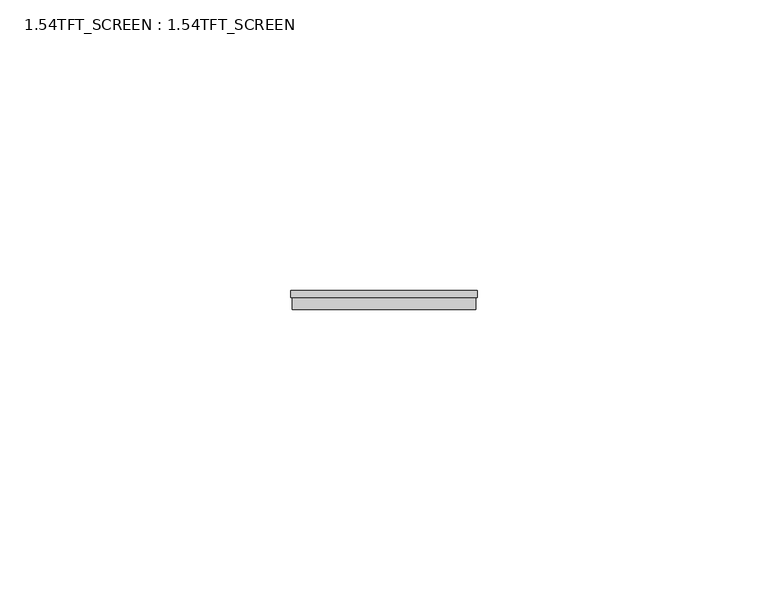
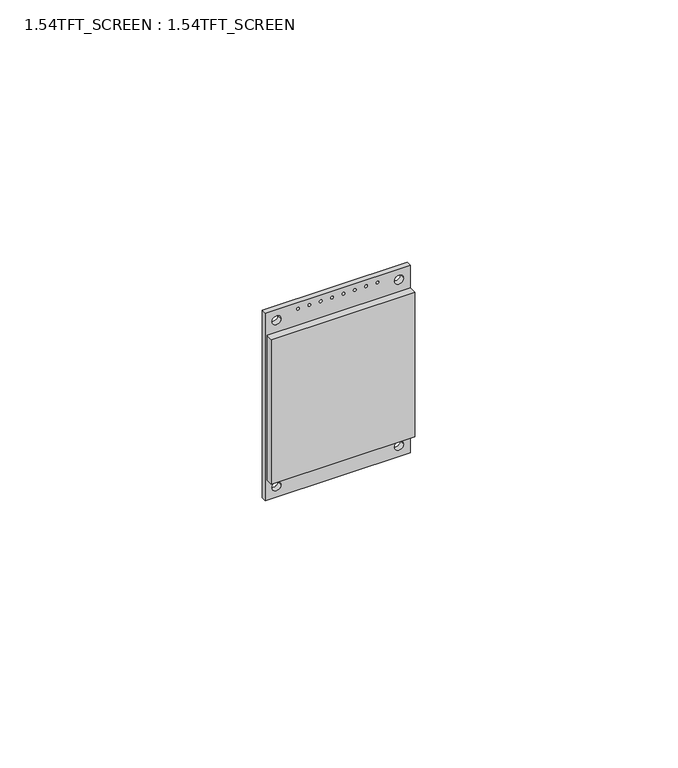
"""IFC4 building model written with IfcOpenShell, lengths in millimetres: furniture geometry, 1.54TFT_SCREEN : 1.54TFT_SCREEN."""

import ifcopenshell
import ifcopenshell.guid

model = None  # the IFC model being written
_history = None  # IfcOwnerHistory: only IFC2X3 demands one
_inside = {}  # id of a spatial element -> (the spatial element, [elements in it])
_under = {}  # id of a project, library or spatial element -> (it, [spatial elements below it])
_declared = {}  # id of a project -> (the project, [libraries it declares])
_typed = {}  # id of a type object -> (the type object, [elements of that type])
_made_of = {}  # id of a material, layer set ... -> (it, [elements and type objects made of it])


def new_model(schema):
    """Start an empty IFC model of exactly this schema.

    Asked for "IFC4X3", IfcOpenShell would pick the latest addendum, in which some entities
    have other attributes; the version numbers below select the first issue.
    IFC2X3 requires an IfcOwnerHistory on every rooted entity: one is made here for all.
    """
    global model, _history
    if schema == "IFC4X3":
        model = ifcopenshell.file(schema_version=(4, 3, 0, 0))
    else:
        model = ifcopenshell.file(schema=schema)
    _inside.clear()
    _under.clear()
    _declared.clear()
    _typed.clear()
    _made_of.clear()
    _history = None
    if model.schema == "IFC2X3":
        org = make("IfcOrganization", Name="unknown")
        user = make(
            "IfcPersonAndOrganization",
            ThePerson=make("IfcPerson", FamilyName="unknown"),
            TheOrganization=org,
        )
        app = make(
            "IfcApplication",
            ApplicationDeveloper=org,
            Version="unknown",
            ApplicationFullName="unknown",
            ApplicationIdentifier="unknown",
        )
        _history = make(
            "IfcOwnerHistory",
            OwningUser=user,
            OwningApplication=app,
            ChangeAction="ADDED",
            CreationDate=0,
        )
    return model


def make(cls, **values):
    """One entity of the class cls with the attributes given. An attribute that is None is left unset."""
    return model.create_entity(
        cls, **{name: value for name, value in values.items() if value is not None}
    )


def rooted(cls, **values):
    """An entity with a GlobalId (a new one), such as an element, a storey or a relation."""
    return make(cls, GlobalId=ifcopenshell.guid.new(), OwnerHistory=_history, **values)


def si_unit(unit_type, name, prefix=None):
    """IfcSIUnit, for example si_unit("LENGTHUNIT", "METRE", prefix="MILLI")."""
    return make("IfcSIUnit", UnitType=unit_type, Prefix=prefix, Name=name)


def assignment(units):
    """IfcUnitAssignment: the units of a project."""
    return None if units is None else make("IfcUnitAssignment", Units=units)


def point(xyz):
    """IfcCartesianPoint."""
    return None if xyz is None else make("IfcCartesianPoint", Coordinates=xyz)


def direction(xyz):
    """IfcDirection."""
    return None if xyz is None else make("IfcDirection", DirectionRatios=xyz)


def frame(location, z_axis=None, x_axis=None):
    """IfcAxis2Placement3D, a coordinate frame: its origin and axes. An axis left out is left unset."""
    return make(
        "IfcAxis2Placement3D",
        Location=point(location),
        Axis=direction(z_axis),
        RefDirection=direction(x_axis),
    )


def frame_2d(location, x_axis=None):
    """IfcAxis2Placement2D, a coordinate frame in the plane: its origin and x axis."""
    return make(
        "IfcAxis2Placement2D", Location=point(location), RefDirection=direction(x_axis)
    )


def origin():
    """The frame at (0, 0, 0) with its axes left unset."""
    return frame((0.0, 0.0, 0.0))


def place(relative_to, where):
    """IfcLocalPlacement: puts the frame where relative to a parent placement (None: the world)."""
    return make(
        "IfcLocalPlacement", PlacementRelTo=relative_to, RelativePlacement=where
    )


def context(
    kind, dimensions, precision=None, world=None, true_north=None, identifier=None
):
    """IfcGeometricRepresentationContext, for example the 3D "Model" context."""
    return make(
        "IfcGeometricRepresentationContext",
        ContextIdentifier=identifier,
        ContextType=kind,
        CoordinateSpaceDimension=dimensions,
        Precision=precision,
        WorldCoordinateSystem=world,
        TrueNorth=true_north,
    )


def project(units=None, contexts=None):
    """IfcProject with its units and contexts."""
    return rooted(
        "IfcProject",
        Name="project",
        RepresentationContexts=contexts,
        UnitsInContext=assignment(units),
    )


def spatial(cls, under=None, at=None, **own):
    """A site, building, storey or space (cls), placed at a placement, below another one or the project."""
    s = rooted(cls, ObjectPlacement=at, **own)
    if under is not None:
        _under.setdefault(under.id(), (under, []))[1].append(s)
    return s


def polyline(points):
    """IfcPolyline through the points."""
    return make("IfcPolyline", Points=[point(p) for p in points])


def circle_curve(where, radius):
    """IfcCircle in the frame where."""
    return make("IfcCircle", Position=where, Radius=radius)


def trimmed(basis, trim1, trim2, sense, master):
    """IfcTrimmedCurve: the piece of a basis curve between two trims."""
    return make(
        "IfcTrimmedCurve",
        BasisCurve=basis,
        Trim1=trim1,
        Trim2=trim2,
        SenseAgreement=sense,
        MasterRepresentation=master,
    )


def segment(curve, same_sense, transition):
    """IfcCompositeCurveSegment."""
    return make(
        "IfcCompositeCurveSegment",
        Transition=transition,
        SameSense=same_sense,
        ParentCurve=curve,
    )


def composite_curve(segments, self_intersect=None):
    """IfcCompositeCurve: segments joined end to end."""
    return make("IfcCompositeCurve", Segments=segments, SelfIntersect=self_intersect)


def outline(outer, holes=None, kind="AREA"):
    """IfcArbitraryClosedProfileDef: a profile drawn as a closed curve; with holes, ...WithVoids."""
    if holes is None:
        return make("IfcArbitraryClosedProfileDef", ProfileType=kind, OuterCurve=outer)
    return make(
        "IfcArbitraryProfileDefWithVoids",
        ProfileType=kind,
        OuterCurve=outer,
        InnerCurves=holes,
    )


def extrude(swept, where, along, depth):
    """IfcExtrudedAreaSolid: the profile swept, set in the frame where, extruded along a direction by depth."""
    return make(
        "IfcExtrudedAreaSolid",
        SweptArea=swept,
        Position=where,
        ExtrudedDirection=direction(along),
        Depth=depth,
    )


def shape(context_of_items, identifier, shape_type, items):
    """IfcShapeRepresentation: the items that make up one representation, for example the "Body"."""
    return make(
        "IfcShapeRepresentation",
        ContextOfItems=context_of_items,
        RepresentationIdentifier=identifier,
        RepresentationType=shape_type,
        Items=items,
    )


def source(mapping_origin, context_of_items, identifier, shape_type, items):
    """IfcRepresentationMap: a shape defined once, which mapped items show again and again."""
    return make(
        "IfcRepresentationMap",
        MappingOrigin=mapping_origin,
        MappedRepresentation=shape(context_of_items, identifier, shape_type, items),
    )


def transform(
    local_origin,
    x_axis=None,
    y_axis=None,
    z_axis=None,
    scale=None,
    scale2=None,
    scale3=None,
    uniform=True,
):
    """IfcCartesianTransformationOperator3D, or its non-uniform kind. x_axis, y_axis, z_axis: its Axis1, 2, 3."""
    if uniform:
        return make(
            "IfcCartesianTransformationOperator3D",
            Axis1=direction(x_axis),
            Axis2=direction(y_axis),
            LocalOrigin=point(local_origin),
            Scale=scale,
            Axis3=direction(z_axis),
        )
    return make(
        "IfcCartesianTransformationOperator3DnonUniform",
        Axis1=direction(x_axis),
        Axis2=direction(y_axis),
        LocalOrigin=point(local_origin),
        Scale=scale,
        Axis3=direction(z_axis),
        Scale2=scale2,
        Scale3=scale3,
    )


def mapped(mapping_source, mapping_target):
    """IfcMappedItem: shows the shape of a source again, moved by a transform."""
    return make(
        "IfcMappedItem", MappingSource=mapping_source, MappingTarget=mapping_target
    )


def made_of(thing, what):
    """Note that an element or type object is made of a material, layer set ...; save() writes the relation."""
    if what is not None:
        _made_of.setdefault(what.id(), (what, []))[1].append(thing)
    return thing


def element(
    cls,
    number,
    at=None,
    inside=None,
    cuts=None,
    type_object=None,
    material=None,
    context=None,
    identifier="Body",
    shape_type=None,
    held_by="IfcProductDefinitionShape",
    body=None,
    shapes=None,
    **own,
):
    """One element of the class cls, such as IfcWall. Its Tag is "e" and its number.

    at: its placement. inside: the storey or other place that contains it. cuts: it is an
    opening in that element (IfcRelVoidsElement). A single representation is given by context,
    identifier, shape_type and body (its items); several are given by shapes. held_by: the class
    of the entity that holds the representations. save() writes the other relations.
    """
    e = rooted(cls, Tag="e%d" % number, ObjectPlacement=at, **own)
    if body is not None:
        shapes = [shape(context, identifier, shape_type, body)]
    if shapes is not None:
        e.Representation = make(held_by, Representations=shapes)
    if inside is not None:
        _inside.setdefault(inside.id(), (inside, []))[1].append(e)
    if cuts is not None:
        rooted(
            "IfcRelVoidsElement", RelatingBuildingElement=cuts, RelatedOpeningElement=e
        )
    if type_object is not None:
        _typed.setdefault(type_object.id(), (type_object, []))[1].append(e)
    return made_of(e, material)


def aggregate(whole, parts):
    """IfcRelAggregates: a whole, such as a stair, and the parts it consists of."""
    return rooted("IfcRelAggregates", RelatingObject=whole, RelatedObjects=parts)


def save(model, path):
    """Write the relations noted so far, then the file.

    IfcRelAggregates (storeys below a building ...), IfcRelContainedInSpatialStructure (elements
    in a storey), IfcRelDefinesByType, IfcRelAssociatesMaterial and IfcRelDeclares: one each for
    every whole, place, type object, material and project.
    """
    for whole, parts in _under.values():
        aggregate(whole, parts)
    for where, things in _inside.values():
        rooted(
            "IfcRelContainedInSpatialStructure",
            RelatedElements=things,
            RelatingStructure=where,
        )
    for kind, things in _typed.values():
        rooted("IfcRelDefinesByType", RelatedObjects=things, RelatingType=kind)
    for what, things in _made_of.values():
        rooted("IfcRelAssociatesMaterial", RelatedObjects=things, RelatingMaterial=what)
    for by, libraries in _declared.values():
        rooted("IfcRelDeclares", RelatingContext=by, RelatedDefinitions=libraries)
    model.write(path)


def furniture_1_54tft_screen_1_54tft_screen_d9e98271(model_context):
    return source(origin(), model_context, "Body", "SweptSolid", [
        extrude(outline(polyline([(43.7, 16.0), (43.7, -16.0), (0.0, -16.0), (0.0, 16.0), (43.7, 16.0)]), holes=[composite_curve([segment(trimmed(circle_curve(frame_2d((2.5, 13.5)), 1.0), [point((2.5, 14.5))], [point((2.5, 12.5))], True, "CARTESIAN"), True, "CONTINUOUS"), segment(trimmed(circle_curve(frame_2d((2.5, 13.5)), 1.0), [point((2.5, 12.5))], [point((2.5, 14.5))], True, "CARTESIAN"), True, "CONTINUOUS")], self_intersect=False), composite_curve([segment(trimmed(circle_curve(frame_2d((41.2, 13.5)), 1.0), [point((41.2, 14.5))], [point((41.2, 12.5))], True, "CARTESIAN"), True, "CONTINUOUS"), segment(trimmed(circle_curve(frame_2d((41.2, 13.5)), 1.0), [point((41.2, 12.5))], [point((41.2, 14.5))], True, "CARTESIAN"), True, "CONTINUOUS")], self_intersect=False), composite_curve([segment(trimmed(circle_curve(frame_2d((42.2, -1.25)), 0.3), [point((42.2, -0.95))], [point((42.2, -1.55))], True, "CARTESIAN"), True, "CONTINUOUS"), segment(trimmed(circle_curve(frame_2d((42.2, -1.25)), 0.3), [point((42.2, -1.55))], [point((42.2, -0.95))], True, "CARTESIAN"), True, "CONTINUOUS")], self_intersect=False), composite_curve([segment(trimmed(circle_curve(frame_2d((42.2, 1.25)), 0.3), [point((42.2, 1.55))], [point((42.2, 0.95))], True, "CARTESIAN"), True, "CONTINUOUS"), segment(trimmed(circle_curve(frame_2d((42.2, 1.25)), 0.3), [point((42.2, 0.95))], [point((42.2, 1.55))], True, "CARTESIAN"), True, "CONTINUOUS")], self_intersect=False), composite_curve([segment(trimmed(circle_curve(frame_2d((42.2, 3.75)), 0.3), [point((42.2, 4.05))], [point((42.2, 3.45))], True, "CARTESIAN"), True, "CONTINUOUS"), segment(trimmed(circle_curve(frame_2d((42.2, 3.75)), 0.3), [point((42.2, 3.45))], [point((42.2, 4.05))], True, "CARTESIAN"), True, "CONTINUOUS")], self_intersect=False), composite_curve([segment(trimmed(circle_curve(frame_2d((42.2, 6.25)), 0.3), [point((42.2, 6.55))], [point((42.2, 5.95))], True, "CARTESIAN"), True, "CONTINUOUS"), segment(trimmed(circle_curve(frame_2d((42.2, 6.25)), 0.3), [point((42.2, 5.95))], [point((42.2, 6.55))], True, "CARTESIAN"), True, "CONTINUOUS")], self_intersect=False), composite_curve([segment(trimmed(circle_curve(frame_2d((42.2, 8.75)), 0.3), [point((42.2, 9.05))], [point((42.2, 8.45))], True, "CARTESIAN"), True, "CONTINUOUS"), segment(trimmed(circle_curve(frame_2d((42.2, 8.75)), 0.3), [point((42.2, 8.45))], [point((42.2, 9.05))], True, "CARTESIAN"), True, "CONTINUOUS")], self_intersect=False), composite_curve([segment(trimmed(circle_curve(frame_2d((42.2, -3.75)), 0.3), [point((42.2, -3.45))], [point((42.2, -4.05))], True, "CARTESIAN"), True, "CONTINUOUS"), segment(trimmed(circle_curve(frame_2d((42.2, -3.75)), 0.3), [point((42.2, -4.05))], [point((42.2, -3.45))], True, "CARTESIAN"), True, "CONTINUOUS")], self_intersect=False), composite_curve([segment(trimmed(circle_curve(frame_2d((42.2, -6.25)), 0.3), [point((42.2, -5.95))], [point((42.2, -6.55))], True, "CARTESIAN"), True, "CONTINUOUS"), segment(trimmed(circle_curve(frame_2d((42.2, -6.25)), 0.3), [point((42.2, -6.55))], [point((42.2, -5.95))], True, "CARTESIAN"), True, "CONTINUOUS")], self_intersect=False), composite_curve([segment(trimmed(circle_curve(frame_2d((42.2, -8.75)), 0.3), [point((42.2, -8.45))], [point((42.2, -9.05))], True, "CARTESIAN"), True, "CONTINUOUS"), segment(trimmed(circle_curve(frame_2d((42.2, -8.75)), 0.3), [point((42.2, -9.05))], [point((42.2, -8.45))], True, "CARTESIAN"), True, "CONTINUOUS")], self_intersect=False), composite_curve([segment(trimmed(circle_curve(frame_2d((41.2, -13.5)), 1.0), [point((41.2, -14.5))], [point((41.2, -12.5))], True, "CARTESIAN"), True, "CONTINUOUS"), segment(trimmed(circle_curve(frame_2d((41.2, -13.5)), 1.0), [point((41.2, -12.5))], [point((41.2, -14.5))], True, "CARTESIAN"), True, "CONTINUOUS")], self_intersect=False), composite_curve([segment(trimmed(circle_curve(frame_2d((2.5, -13.5)), 1.0), [point((2.5, -14.5))], [point((2.5, -12.5))], True, "CARTESIAN"), True, "CONTINUOUS"), segment(trimmed(circle_curve(frame_2d((2.5, -13.5)), 1.0), [point((2.5, -12.5))], [point((2.5, -14.5))], True, "CARTESIAN"), True, "CONTINUOUS")], self_intersect=False)]), frame((0.0, -1.2, 0.0), z_axis=(0.0, 1.0, 0.0), x_axis=(0.0, 0.0, 1.0)), (0.0, 0.0, 1.0), 1.2),
        extrude(outline(polyline([(15.76, -1.3), (15.76, -3.2), (-15.76, -3.2), (-15.76, -1.3), (15.76, -1.3)])), frame((0.0, 0.0, 5.0), z_axis=(0.0, 0.0, 1.0), x_axis=(1.0, 0.0, 0.0)), (0.0, 0.0, 1.0), 33.7),
        extrude(outline(polyline([(13.86, -2.3592442), (13.86, -3.2), (-13.86, -3.2), (-13.86, -2.3592442), (13.86, -2.3592442)])), frame((0.0, 0.0, 9.5994076), z_axis=(0.0, 0.0, 1.0), x_axis=(1.0, 0.0, 0.0)), (0.0, 0.0, 1.0), 27.7),
    ])


if __name__ == "__main__":
    model = new_model("IFC4")
    model_context = context("Model", 3, world=origin())
    ifc_project = project(units=[si_unit("LENGTHUNIT", "METRE", prefix="MILLI")], contexts=[model_context])
    site = spatial("IfcSite", under=ifc_project)
    building = spatial("IfcBuilding", under=site)
    placement = place(None, origin())
    furniture_1_54tft_screen_1_54tft_screen_shape = furniture_1_54tft_screen_1_54tft_screen_d9e98271(model_context)
    element("IfcFurniture", 1, ObjectType="1.54TFT_SCREEN : 1.54TFT_SCREEN", at=placement, inside=building, context=model_context, shape_type="MappedRepresentation", body=[
        mapped(furniture_1_54tft_screen_1_54tft_screen_shape, transform((0.0, 0.0, 0.0), x_axis=(1.0, 0.0, 0.0), y_axis=(0.0, 1.0, 0.0), z_axis=(0.0, 0.0, 1.0))),
    ])
    save(model, "model.ifc")

# Revit data of these elements
# Type "1.54TFT_SCREEN : 1.54TFT_SCREEN"
#   Default Elevation = 0
# Element 1 (IfcFurniture, "1.54TFT_SCREEN : 1.54TFT_SCREEN")
#   Materials on its faces: ".VIDRO"
# Materials
#   ".VIDRO": class "Vidro", colour RGB 165 190 164, transparency 0.4, Cost = 0
